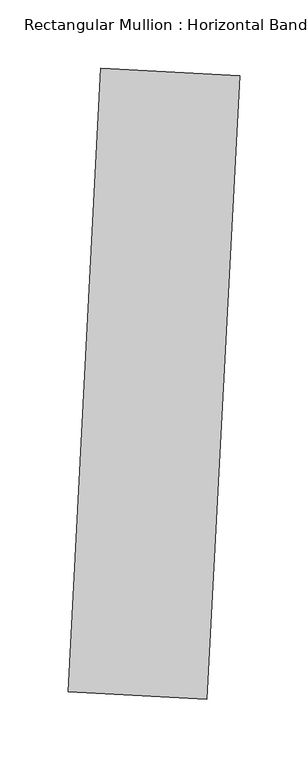
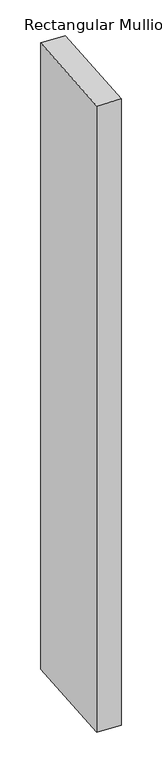
"""IFC4 building model written with IfcOpenShell, lengths in millimetres: member geometry, Rectangular Mullion : Horizontal Band."""

from ifc_helpers import new_model, si_unit, frame, origin, place, context, project, spatial, polyline, outline, extrude, source, transform, mapped, element, save


def rectangular_mullion_horizontal_band_291f11ce(model_context):
    return source(origin(), model_context, "Body", "SweptSolid", [
        extrude(outline(polyline([(62.69438, 301.8280451), (38.7663808, -154.7453782), (-62.69438, -149.4280451), (-38.7663808, 307.1453782), (62.69438, 301.8280451)])), frame((0.0, 0.0, -2820.8179936), z_axis=(0.0, 0.0, 1.0), x_axis=(1.0, 0.0, 0.0)), (0.0, 0.0, 1.0), 2820.8179936),
    ])


if __name__ == "__main__":
    model = new_model("IFC4")
    model_context = context("Model", 3, world=origin())
    ifc_project = project(units=[si_unit("LENGTHUNIT", "METRE", prefix="MILLI")], contexts=[model_context])
    site = spatial("IfcSite", under=ifc_project)
    building = spatial("IfcBuilding", under=site)
    placement = place(None, origin())
    rectangular_mullion_horizontal_band_shape = rectangular_mullion_horizontal_band_291f11ce(model_context)
    element("IfcMember", 1, ObjectType="Rectangular Mullion : Horizontal Band", at=placement, inside=building, context=model_context, shape_type="MappedRepresentation", body=[
        mapped(rectangular_mullion_horizontal_band_shape, transform((0.0, 0.0, 0.0), x_axis=(1.0, 0.0, 0.0), y_axis=(0.0, 1.0, 0.0), z_axis=(0.0, 0.0, 1.0))),
    ])
    save(model, "model.ifc")

# Revit data of these elements
# Type "Rectangular Mullion : Horizontal Band"
#   built-in parameter 1007351 = 0.25 (stored number, unit not read)
#   built-in parameter 1007304 = 1.5 (stored number, unit not read)
#   built-in parameter 1007301 = 0.166667 (stored number, unit not read)
#   built-in parameter 1007300 = 0.166667 (stored number, unit not read)
# Element 1 (IfcMember, "Rectangular Mullion : Horizontal Band")
#   Materials on its faces: "Aluminum"
# Materials
#   "Aluminum": class "Metal", colour RGB 247 247 247, transparency 0, Description = "Aluminum 6061", Cost = 0
